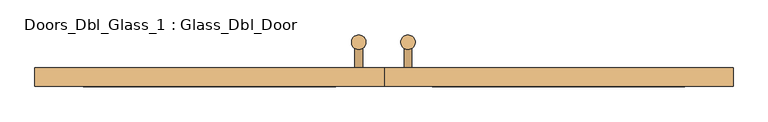
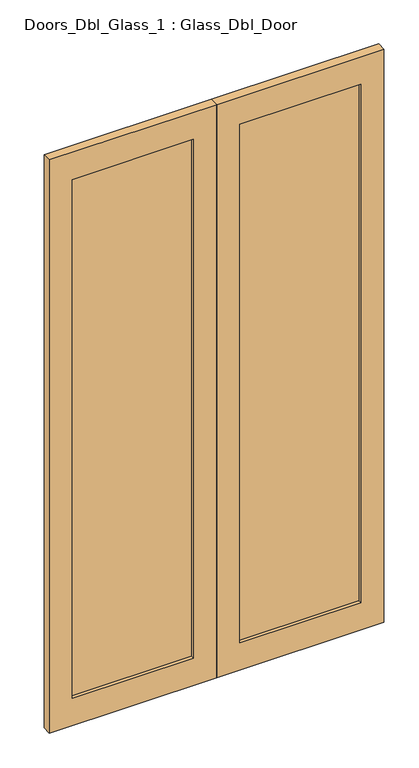
"""IFC4 building model written with IfcOpenShell, lengths in millimetres: door geometry, Doors_Dbl_Glass_1 : Glass_Dbl_Door."""

import ifcopenshell
import ifcopenshell.guid

model = None  # the IFC model being written
_history = None  # IfcOwnerHistory: only IFC2X3 demands one
_inside = {}  # id of a spatial element -> (the spatial element, [elements in it])
_under = {}  # id of a project, library or spatial element -> (it, [spatial elements below it])
_declared = {}  # id of a project -> (the project, [libraries it declares])
_typed = {}  # id of a type object -> (the type object, [elements of that type])
_made_of = {}  # id of a material, layer set ... -> (it, [elements and type objects made of it])


def new_model(schema):
    """Start an empty IFC model of exactly this schema.

    Asked for "IFC4X3", IfcOpenShell would pick the latest addendum, in which some entities
    have other attributes; the version numbers below select the first issue.
    IFC2X3 requires an IfcOwnerHistory on every rooted entity: one is made here for all.
    """
    global model, _history
    if schema == "IFC4X3":
        model = ifcopenshell.file(schema_version=(4, 3, 0, 0))
    else:
        model = ifcopenshell.file(schema=schema)
    _inside.clear()
    _under.clear()
    _declared.clear()
    _typed.clear()
    _made_of.clear()
    _history = None
    if model.schema == "IFC2X3":
        org = make("IfcOrganization", Name="unknown")
        user = make(
            "IfcPersonAndOrganization",
            ThePerson=make("IfcPerson", FamilyName="unknown"),
            TheOrganization=org,
        )
        app = make(
            "IfcApplication",
            ApplicationDeveloper=org,
            Version="unknown",
            ApplicationFullName="unknown",
            ApplicationIdentifier="unknown",
        )
        _history = make(
            "IfcOwnerHistory",
            OwningUser=user,
            OwningApplication=app,
            ChangeAction="ADDED",
            CreationDate=0,
        )
    return model


def make(cls, **values):
    """One entity of the class cls with the attributes given. An attribute that is None is left unset."""
    return model.create_entity(
        cls, **{name: value for name, value in values.items() if value is not None}
    )


def rooted(cls, **values):
    """An entity with a GlobalId (a new one), such as an element, a storey or a relation."""
    return make(cls, GlobalId=ifcopenshell.guid.new(), OwnerHistory=_history, **values)


def si_unit(unit_type, name, prefix=None):
    """IfcSIUnit, for example si_unit("LENGTHUNIT", "METRE", prefix="MILLI")."""
    return make("IfcSIUnit", UnitType=unit_type, Prefix=prefix, Name=name)


def assignment(units):
    """IfcUnitAssignment: the units of a project."""
    return None if units is None else make("IfcUnitAssignment", Units=units)


def point(xyz):
    """IfcCartesianPoint."""
    return None if xyz is None else make("IfcCartesianPoint", Coordinates=xyz)


def direction(xyz):
    """IfcDirection."""
    return None if xyz is None else make("IfcDirection", DirectionRatios=xyz)


def frame(location, z_axis=None, x_axis=None):
    """IfcAxis2Placement3D, a coordinate frame: its origin and axes. An axis left out is left unset."""
    return make(
        "IfcAxis2Placement3D",
        Location=point(location),
        Axis=direction(z_axis),
        RefDirection=direction(x_axis),
    )


def frame_2d(location, x_axis=None):
    """IfcAxis2Placement2D, a coordinate frame in the plane: its origin and x axis."""
    return make(
        "IfcAxis2Placement2D", Location=point(location), RefDirection=direction(x_axis)
    )


def origin():
    """The frame at (0, 0, 0) with its axes left unset."""
    return frame((0.0, 0.0, 0.0))


def place(relative_to, where):
    """IfcLocalPlacement: puts the frame where relative to a parent placement (None: the world)."""
    return make(
        "IfcLocalPlacement", PlacementRelTo=relative_to, RelativePlacement=where
    )


def context(
    kind, dimensions, precision=None, world=None, true_north=None, identifier=None
):
    """IfcGeometricRepresentationContext, for example the 3D "Model" context."""
    return make(
        "IfcGeometricRepresentationContext",
        ContextIdentifier=identifier,
        ContextType=kind,
        CoordinateSpaceDimension=dimensions,
        Precision=precision,
        WorldCoordinateSystem=world,
        TrueNorth=true_north,
    )


def project(units=None, contexts=None):
    """IfcProject with its units and contexts."""
    return rooted(
        "IfcProject",
        Name="project",
        RepresentationContexts=contexts,
        UnitsInContext=assignment(units),
    )


def spatial(cls, under=None, at=None, **own):
    """A site, building, storey or space (cls), placed at a placement, below another one or the project."""
    s = rooted(cls, ObjectPlacement=at, **own)
    if under is not None:
        _under.setdefault(under.id(), (under, []))[1].append(s)
    return s


def polyline(points):
    """IfcPolyline through the points."""
    return make("IfcPolyline", Points=[point(p) for p in points])


def circle_curve(where, radius):
    """IfcCircle in the frame where."""
    return make("IfcCircle", Position=where, Radius=radius)


def trimmed(basis, trim1, trim2, sense, master):
    """IfcTrimmedCurve: the piece of a basis curve between two trims."""
    return make(
        "IfcTrimmedCurve",
        BasisCurve=basis,
        Trim1=trim1,
        Trim2=trim2,
        SenseAgreement=sense,
        MasterRepresentation=master,
    )


def segment(curve, same_sense, transition):
    """IfcCompositeCurveSegment."""
    return make(
        "IfcCompositeCurveSegment",
        Transition=transition,
        SameSense=same_sense,
        ParentCurve=curve,
    )


def composite_curve(segments, self_intersect=None):
    """IfcCompositeCurve: segments joined end to end."""
    return make("IfcCompositeCurve", Segments=segments, SelfIntersect=self_intersect)


def outline(outer, holes=None, kind="AREA"):
    """IfcArbitraryClosedProfileDef: a profile drawn as a closed curve; with holes, ...WithVoids."""
    if holes is None:
        return make("IfcArbitraryClosedProfileDef", ProfileType=kind, OuterCurve=outer)
    return make(
        "IfcArbitraryProfileDefWithVoids",
        ProfileType=kind,
        OuterCurve=outer,
        InnerCurves=holes,
    )


def extrude(swept, where, along, depth):
    """IfcExtrudedAreaSolid: the profile swept, set in the frame where, extruded along a direction by depth."""
    return make(
        "IfcExtrudedAreaSolid",
        SweptArea=swept,
        Position=where,
        ExtrudedDirection=direction(along),
        Depth=depth,
    )


def shape(context_of_items, identifier, shape_type, items):
    """IfcShapeRepresentation: the items that make up one representation, for example the "Body"."""
    return make(
        "IfcShapeRepresentation",
        ContextOfItems=context_of_items,
        RepresentationIdentifier=identifier,
        RepresentationType=shape_type,
        Items=items,
    )


def source(mapping_origin, context_of_items, identifier, shape_type, items):
    """IfcRepresentationMap: a shape defined once, which mapped items show again and again."""
    return make(
        "IfcRepresentationMap",
        MappingOrigin=mapping_origin,
        MappedRepresentation=shape(context_of_items, identifier, shape_type, items),
    )


def transform(
    local_origin,
    x_axis=None,
    y_axis=None,
    z_axis=None,
    scale=None,
    scale2=None,
    scale3=None,
    uniform=True,
):
    """IfcCartesianTransformationOperator3D, or its non-uniform kind. x_axis, y_axis, z_axis: its Axis1, 2, 3."""
    if uniform:
        return make(
            "IfcCartesianTransformationOperator3D",
            Axis1=direction(x_axis),
            Axis2=direction(y_axis),
            LocalOrigin=point(local_origin),
            Scale=scale,
            Axis3=direction(z_axis),
        )
    return make(
        "IfcCartesianTransformationOperator3DnonUniform",
        Axis1=direction(x_axis),
        Axis2=direction(y_axis),
        LocalOrigin=point(local_origin),
        Scale=scale,
        Axis3=direction(z_axis),
        Scale2=scale2,
        Scale3=scale3,
    )


def mapped(mapping_source, mapping_target):
    """IfcMappedItem: shows the shape of a source again, moved by a transform."""
    return make(
        "IfcMappedItem", MappingSource=mapping_source, MappingTarget=mapping_target
    )


def made_of(thing, what):
    """Note that an element or type object is made of a material, layer set ...; save() writes the relation."""
    if what is not None:
        _made_of.setdefault(what.id(), (what, []))[1].append(thing)
    return thing


def element(
    cls,
    number,
    at=None,
    inside=None,
    cuts=None,
    type_object=None,
    material=None,
    context=None,
    identifier="Body",
    shape_type=None,
    held_by="IfcProductDefinitionShape",
    body=None,
    shapes=None,
    **own,
):
    """One element of the class cls, such as IfcWall. Its Tag is "e" and its number.

    at: its placement. inside: the storey or other place that contains it. cuts: it is an
    opening in that element (IfcRelVoidsElement). A single representation is given by context,
    identifier, shape_type and body (its items); several are given by shapes. held_by: the class
    of the entity that holds the representations. save() writes the other relations.
    """
    e = rooted(cls, Tag="e%d" % number, ObjectPlacement=at, **own)
    if body is not None:
        shapes = [shape(context, identifier, shape_type, body)]
    if shapes is not None:
        e.Representation = make(held_by, Representations=shapes)
    if inside is not None:
        _inside.setdefault(inside.id(), (inside, []))[1].append(e)
    if cuts is not None:
        rooted(
            "IfcRelVoidsElement", RelatingBuildingElement=cuts, RelatedOpeningElement=e
        )
    if type_object is not None:
        _typed.setdefault(type_object.id(), (type_object, []))[1].append(e)
    return made_of(e, material)


def aggregate(whole, parts):
    """IfcRelAggregates: a whole, such as a stair, and the parts it consists of."""
    return rooted("IfcRelAggregates", RelatingObject=whole, RelatedObjects=parts)


def save(model, path):
    """Write the relations noted so far, then the file.

    IfcRelAggregates (storeys below a building ...), IfcRelContainedInSpatialStructure (elements
    in a storey), IfcRelDefinesByType, IfcRelAssociatesMaterial and IfcRelDeclares: one each for
    every whole, place, type object, material and project.
    """
    for whole, parts in _under.values():
        aggregate(whole, parts)
    for where, things in _inside.values():
        rooted(
            "IfcRelContainedInSpatialStructure",
            RelatedElements=things,
            RelatingStructure=where,
        )
    for kind, things in _typed.values():
        rooted("IfcRelDefinesByType", RelatedObjects=things, RelatingType=kind)
    for what, things in _made_of.values():
        rooted("IfcRelAssociatesMaterial", RelatedObjects=things, RelatingMaterial=what)
    for by, libraries in _declared.values():
        rooted("IfcRelDeclares", RelatingContext=by, RelatedDefinitions=libraries)
    model.write(path)


def doors_dbl_glass_1_glass_dbl_door_2c6c785a(model_context):
    return source(origin(), model_context, "Body", "SweptSolid", [
        extrude(outline(composite_curve([segment(trimmed(circle_curve(frame_2d((49.6069979, 116.0715804)), 15.0), [point((49.6069979, 101.0715804))], [point((49.6069979, 131.0715804))], False, "CARTESIAN"), True, "CONTINUOUS"), segment(trimmed(circle_curve(frame_2d((49.6069979, 116.0715804)), 15.0), [point((49.6069979, 131.0715804))], [point((49.6069979, 101.0715804))], False, "CARTESIAN"), True, "CONTINUOUS")], self_intersect=False)), frame((0.0, 0.0, 650.0), z_axis=(0.0, 0.0, 1.0), x_axis=(1.0, 0.0, 0.0)), (0.0, 0.0, 1.0), 900.0),
        extrude(outline(composite_curve([segment(trimmed(circle_curve(frame_2d((-52.537897, 116.0715804)), 15.0), [point((-52.537897, 101.0715804))], [point((-52.537897, 131.0715804))], False, "CARTESIAN"), True, "CONTINUOUS"), segment(trimmed(circle_curve(frame_2d((-52.537897, 116.0715804)), 15.0), [point((-52.537897, 131.0715804))], [point((-52.537897, 101.0715804))], False, "CARTESIAN"), True, "CONTINUOUS")], self_intersect=False)), frame((0.0, 0.0, 650.0), z_axis=(0.0, 0.0, 1.0), x_axis=(1.0, 0.0, 0.0)), (0.0, 0.0, 1.0), 900.0),
        extrude(outline(composite_curve([segment(trimmed(circle_curve(frame_2d((750.0, 49.6069979)), 8.0), [point((750.0, 57.6069979))], [point((750.0, 41.6069979))], False, "CARTESIAN"), True, "CONTINUOUS"), segment(trimmed(circle_curve(frame_2d((750.0, 49.6069979)), 8.0), [point((750.0, 41.6069979))], [point((750.0, 57.6069979))], False, "CARTESIAN"), True, "CONTINUOUS")], self_intersect=False)), frame((0.0, 62.5788556, 0.0), z_axis=(0.0, 1.0, 0.0), x_axis=(0.0, 0.0, 1.0)), (0.0, 0.0, 1.0), 53.4927248),
        extrude(outline(composite_curve([segment(trimmed(circle_curve(frame_2d((750.0, -52.537897)), 8.0), [point((750.0, -44.537897))], [point((750.0, -60.537897))], False, "CARTESIAN"), True, "CONTINUOUS"), segment(trimmed(circle_curve(frame_2d((750.0, -52.537897)), 8.0), [point((750.0, -60.537897))], [point((750.0, -44.537897))], False, "CARTESIAN"), True, "CONTINUOUS")], self_intersect=False)), frame((0.0, 62.5788556, 0.0), z_axis=(0.0, 1.0, 0.0), x_axis=(0.0, 0.0, 1.0)), (0.0, 0.0, 1.0), 53.4927248),
        extrude(outline(composite_curve([segment(trimmed(circle_curve(frame_2d((1450.0, 49.6069979)), 8.0), [point((1450.0, 57.6069979))], [point((1450.0, 41.6069979))], False, "CARTESIAN"), True, "CONTINUOUS"), segment(trimmed(circle_curve(frame_2d((1450.0, 49.6069979)), 8.0), [point((1450.0, 41.6069979))], [point((1450.0, 57.6069979))], False, "CARTESIAN"), True, "CONTINUOUS")], self_intersect=False)), frame((0.0, 62.5788556, 0.0), z_axis=(0.0, 1.0, 0.0), x_axis=(0.0, 0.0, 1.0)), (0.0, 0.0, 1.0), 53.4927248),
        extrude(outline(composite_curve([segment(trimmed(circle_curve(frame_2d((1450.0, -52.537897)), 8.0), [point((1450.0, -44.537897))], [point((1450.0, -60.537897))], False, "CARTESIAN"), True, "CONTINUOUS"), segment(trimmed(circle_curve(frame_2d((1450.0, -52.537897)), 8.0), [point((1450.0, -60.537897))], [point((1450.0, -44.537897))], False, "CARTESIAN"), True, "CONTINUOUS")], self_intersect=False)), frame((0.0, 62.5788556, 0.0), z_axis=(0.0, 1.0, 0.0), x_axis=(0.0, 0.0, 1.0)), (0.0, 0.0, 1.0), 53.4927248),
        extrude(outline(polyline([(2625.0, -724.9999999), (0.0, -724.9999999), (0.0, 0.0), (2625.0, 0.0), (2625.0, -724.9999999)]), holes=[polyline([(2500.0, -624.9999999), (2500.0, -100.0), (125.0, -100.0), (125.0, -624.9999999), (2500.0, -624.9999999)])]), frame((0.0, 24.035259, 0.0), z_axis=(0.0, 1.0, 0.0), x_axis=(0.0, 0.0, 1.0)), (0.0, 0.0, 1.0), 38.5435966),
        extrude(outline(polyline([(2625.0, 0.0), (0.0, 0.0), (0.0, 724.9999999), (2625.0, 724.9999999), (2625.0, 0.0)]), holes=[polyline([(2500.0, 100.0), (2500.0, 624.9999999), (125.0, 624.9999999), (125.0, 100.0), (2500.0, 100.0)])]), frame((0.0, 24.035259, 0.0), z_axis=(0.0, 1.0, 0.0), x_axis=(0.0, 0.0, 1.0)), (0.0, 0.0, 1.0), 38.5435966),
        extrude(outline(polyline([(-100.0, 38.0), (-624.9999999, 38.0), (-624.9999999, 50.0), (-100.0, 50.0), (-100.0, 38.0)])), frame((0.0, 0.0, 125.0), z_axis=(0.0, 0.0, 1.0), x_axis=(1.0, 0.0, 0.0)), (0.0, 0.0, 1.0), 2375.0),
        extrude(outline(polyline([(624.9999999, 38.0), (100.0, 38.0), (100.0, 50.0), (624.9999999, 50.0), (624.9999999, 38.0)])), frame((0.0, 0.0, 125.0), z_axis=(0.0, 0.0, 1.0), x_axis=(1.0, 0.0, 0.0)), (0.0, 0.0, 1.0), 2375.0),
    ])


if __name__ == "__main__":
    model = new_model("IFC4")
    model_context = context("Model", 3, world=origin())
    ifc_project = project(units=[si_unit("LENGTHUNIT", "METRE", prefix="MILLI")], contexts=[model_context])
    site = spatial("IfcSite", under=ifc_project)
    building = spatial("IfcBuilding", under=site)
    placement = place(None, origin())
    doors_dbl_glass_1_glass_dbl_door_shape = doors_dbl_glass_1_glass_dbl_door_2c6c785a(model_context)
    element("IfcDoor", 1, ObjectType="Doors_Dbl_Glass_1 : Glass_Dbl_Door", at=placement, inside=building, context=model_context, shape_type="MappedRepresentation", body=[
        mapped(doors_dbl_glass_1_glass_dbl_door_shape, transform((0.0, 0.0, 0.0), x_axis=(1.0, 0.0, 0.0), y_axis=(0.0, 1.0, 0.0), z_axis=(0.0, 0.0, 1.0))),
    ])
    save(model, "model.ifc")

# Revit data of these elements
# Project information
#   Project Issue Date = "Issue Date"
#   Project Status = "Project Status"
#   Client Name = "Owner"
#   Project Address = "Enter address here"
#   Project Name = "Project Name"
#   Project Number = "Project Number"
# Type "Doors_Dbl_Glass_1 : Glass_Dbl_Door"
#   Type Mark = "48"
#   Construction Type Id = "GSP4R"
#   Analytic Construction = "1/8 in Pilkington single glazing"
#   Visual Light Transmittance = 0.9
#   Stile Shutting = 100 mm
#   Stile Hanging = 100 mm
#   Stile - Top Rail = 125 mm
#   Stile - Bottom Rail = 125 mm
#   Solar Heat Gain Coefficient = 0.78
#   Offset = 50 mm
#   Heat Transfer Coefficient (U) = 3.6886 W/(m²·K)
#   Glass Thickness = 12 mm
#   Material Ironmongery = Metal - Aluminum
#   Material Door = Metal - Aluminum
#   Material Glass = Glass
#   Function = (empty or 0)
# Element 1 (IfcDoor, "Doors_Dbl_Glass_1 : Glass_Dbl_Door")
#   Materials on its faces: "Metal - Aluminum", "Glass"
# Materials
#   "Metal - Aluminum": class "Metal", colour RGB 247 247 247, transparency 0
#   "Glass": class "Glass", colour RGB 0 128 192, transparency 0.9, Description = "Soda Lime Glass", Cost = 0
